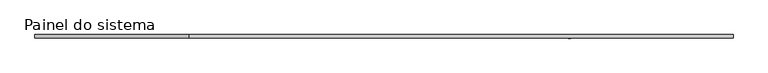
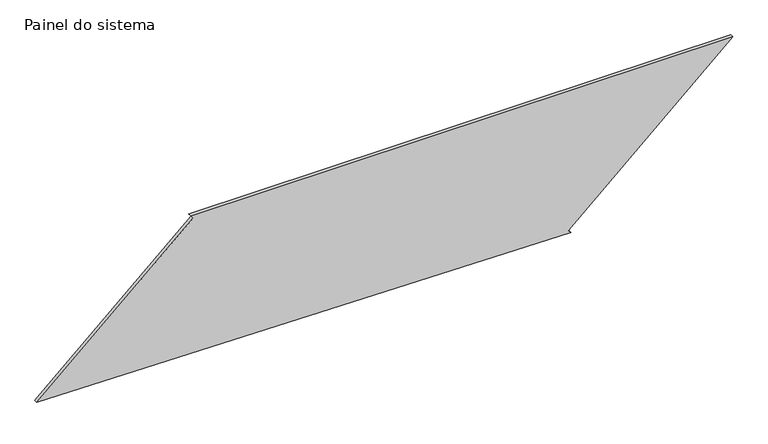
"""IFC4 building model written with IfcOpenShell, lengths in millimetres: plate geometry, Painel do sistema : Envidraçado."""

from ifc_helpers import new_model, si_unit, frame, origin, place, context, project, spatial, polyline, outline, extrude, source, transform, mapped, element, save


def painel_do_sistema_492e67b5(model_context):
    return source(origin(), model_context, "Body", "SweptSolid", [
        extrude(outline(polyline([(0.0, 1309.4232729), (18.5968466, 1292.715272), (1056.3680083, 2447.8068479), (1056.3680083, -1364.182611), (1037.7711616, -1347.4746101), (49.1975382, -2447.8068479), (0.0, 1309.4232729)])), frame((0.0, 24.5, 0.0), z_axis=(0.0, 1.0, 0.0), x_axis=(0.0, 0.0, 1.0)), (0.0, 0.0, 1.0), 25.0),
    ])


if __name__ == "__main__":
    model = new_model("IFC4")
    model_context = context("Model", 3, world=origin())
    ifc_project = project(units=[si_unit("LENGTHUNIT", "METRE", prefix="MILLI")], contexts=[model_context])
    site = spatial("IfcSite", under=ifc_project)
    building = spatial("IfcBuilding", under=site)
    placement = place(None, origin())
    painel_do_sistema_shape = painel_do_sistema_492e67b5(model_context)
    element("IfcPlate", 1, ObjectType="Painel do sistema : Envidraçado", at=placement, inside=building, context=model_context, shape_type="MappedRepresentation", body=[
        mapped(painel_do_sistema_shape, transform((0.0, 0.0, 0.0), x_axis=(1.0, 0.0, 0.0), y_axis=(0.0, 1.0, 0.0), z_axis=(0.0, 0.0, 1.0))),
    ])
    save(model, "model.ifc")

# Revit data of these elements
# Type "Painel do sistema : Envidraçado"
#   Construction Type Id = "GSP4R"
#   Analytic Construction = "Vidraça única Pilkington 1/8 pol"
#   Visual Light Transmittance = 0.9
#   Solar Heat Gain Coefficient = 0.86
#   Heat Transfer Coefficient (U) = 6.7069 W/(m²·K)
# Element 1 (IfcPlate, "Painel do sistema : Envidraçado")
#   Materials on its faces: "Vidro"
# Materials
#   "Vidro": class "Vidro", colour RGB 0 128 192, transparency 0.9, Description = "Vidro de sílica", Cost = 0
